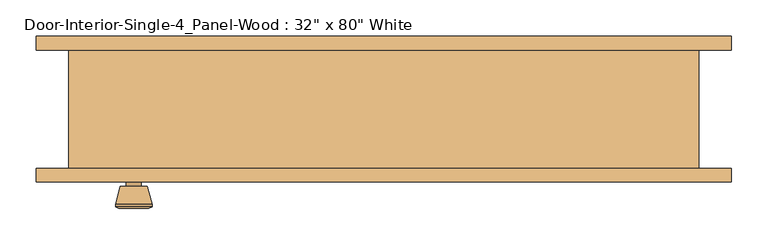
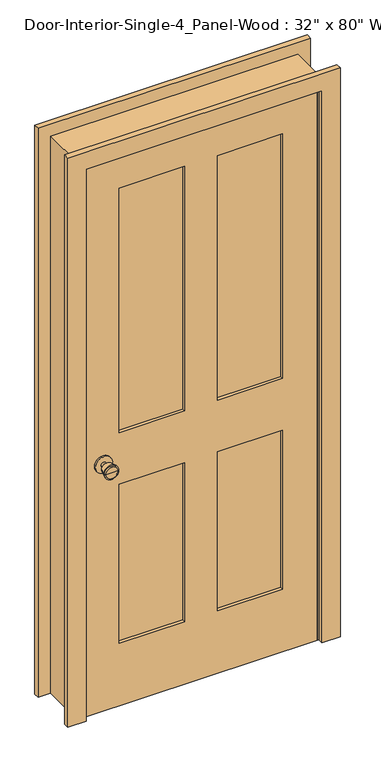
"""IFC4 building model written with IfcOpenShell, lengths in millimetres: door geometry."""

from ifc_helpers import new_model, si_unit, point, frame, frame_2d, origin, place, context, project, spatial, polyline, circle_curve, trimmed, segment, composite_curve, outline, extrude, faceted_brep, source, transform, mapped, element, save
from ifc_brep_helpers import plane_surface, cylinder_surface, revolved_surface, advanced_brep


def door_564574e5(model_context):
    return source(origin(), model_context, "Body", "SolidModel", [
        advanced_brep(
        [(-342.9, -36.8625, 914.4), (-352.9, -36.8625, 914.4), (-332.9, -36.8625, 914.4), (-322.4241324, 12.1375, 914.4), (-363.3758676, 12.1375, 914.4), (-342.9, 12.1375, 914.4), (-317.9, 10.3096319, 914.4), (-367.9, 10.3096319, 914.4), (-317.9, 6.8459537, 914.4), (-367.9, 6.8459537, 914.4), (-324.263764, -17.8625, 914.4), (-361.536236, -17.8625, 914.4), (-332.9, -17.8625, 914.4), (-352.9, -17.8625, 914.4)],
        [
            (0, 1),
            (1, 2, circle_curve(frame((-342.9, -36.8625, 914.4), z_axis=(0.0, -1.0, 0.0), x_axis=(-1.0, 0.0, 0.0)), 10.0)),
            (2, 0),
            (2, 1, circle_curve(frame((-342.9, -36.8625, 914.4), z_axis=(0.0, -1.0, 0.0), x_axis=(-1.0, 0.0, 0.0)), 10.0)),
            (3, 4, circle_curve(frame((-342.9, 12.1375, 914.4), z_axis=(0.0, 1.0, 0.0), x_axis=(-1.0, 0.0, 0.0)), 20.4758676)),
            (4, 5),
            (5, 3),
            (4, 3, circle_curve(frame((-342.9, 12.1375, 914.4), z_axis=(0.0, 1.0, 0.0), x_axis=(-1.0, 0.0, 0.0)), 20.4758676)),
            (6, 7, circle_curve(frame((-342.9, 10.3096319, 914.4), z_axis=(0.0, 1.0, 0.0), x_axis=(-1.0, 0.0, 0.0)), 25.0)),
            (7, 4),
            (3, 6),
            (7, 6, circle_curve(frame((-342.9, 10.3096319, 914.4), z_axis=(0.0, 1.0, 0.0), x_axis=(-1.0, 0.0, 0.0)), 25.0)),
            (8, 9, circle_curve(frame((-342.9, 6.8459537, 914.4), z_axis=(0.0, 1.0, 0.0), x_axis=(-1.0, 0.0, 0.0)), 25.0)),
            (9, 7),
            (6, 8),
            (9, 8, circle_curve(frame((-342.9, 6.8459537, 914.4), z_axis=(0.0, 1.0, 0.0), x_axis=(-1.0, 0.0, 0.0)), 25.0)),
            (10, 11, circle_curve(frame((-342.9, -17.8625, 914.4), z_axis=(0.0, 1.0, 0.0), x_axis=(-1.0, 0.0, 0.0)), 18.636236)),
            (11, 9),
            (8, 10),
            (11, 10, circle_curve(frame((-342.9, -17.8625, 914.4), z_axis=(0.0, 1.0, 0.0), x_axis=(-1.0, 0.0, 0.0)), 18.636236)),
            (12, 13, circle_curve(frame((-342.9, -17.8625, 914.4), z_axis=(0.0, 1.0, 0.0), x_axis=(-1.0, 0.0, 0.0)), 10.0)),
            (13, 11),
            (10, 12),
            (13, 12, circle_curve(frame((-342.9, -17.8625, 914.4), z_axis=(0.0, 1.0, 0.0), x_axis=(-1.0, 0.0, 0.0)), 10.0)),
            (1, 13),
            (12, 2),
        ],
        [
            plane_surface(frame((-342.9, -36.8625, 914.4), z_axis=(0.0, -1.0, 0.0), x_axis=(-1.0, 0.0, 0.0))),
            plane_surface(frame((-342.9, 12.1375, 914.4), z_axis=(0.0, 1.0, 0.0), x_axis=(-1.0, 0.0, 0.0))),
            revolved_surface(polyline([(-363.3758676, 12.1375, 914.4), (-367.9, 10.3096319, 914.4)]), (-342.9, -36.8625, 914.4), (0.0, -1.0, 0.0)),
            cylinder_surface(frame((-342.9, -36.8625, 914.4), z_axis=(0.0, -1.0, 0.0), x_axis=(-1.0, 0.0, 0.0)), 25.0),
            revolved_surface(polyline([(-367.9, 6.8459537, 914.4), (-361.536236, -17.8625, 914.4)]), (-342.9, -36.8625, 914.4), (0.0, -1.0, 0.0)),
            plane_surface(frame((-342.9, -17.8625, 914.4), z_axis=(0.0, -1.0, 0.0), x_axis=(-1.0, 0.0, 0.0))),
            cylinder_surface(frame((-342.9, -36.8625, 914.4), z_axis=(0.0, -1.0, 0.0), x_axis=(-1.0, 0.0, 0.0)), 10.0),
        ],
        [
            (0, [[1, 2, 3]]),
            (0, [[-3, 4, -1]]),
            (1, [[5, 6, 7]]),
            (1, [[8, -7, -6]]),
            (2, [[9, 10, -5, 11]]),
            (2, [[12, -11, -8, -10]]),
            (3, [[13, 14, -9, 15]]),
            (3, [[16, -15, -12, -14]]),
            (4, [[17, 18, -13, 19]]),
            (4, [[20, -19, -16, -18]]),
            (5, [[21, 22, -17, 23]]),
            (5, [[24, -23, -20, -22]]),
            (6, [[-2, 25, -21, 26]]),
            (6, [[-4, -26, -24, -25]]),
        ],
    ),
        extrude(outline(composite_curve([segment(trimmed(circle_curve(frame_2d((914.4, -342.9)), 30.0), [point((914.4, -372.9))], [point((914.4, -312.9))], False, "CARTESIAN"), True, "CONTINUOUS"), segment(trimmed(circle_curve(frame_2d((914.4, -342.9)), 30.0), [point((914.4, -312.9))], [point((914.4, -372.9))], False, "CARTESIAN"), True, "CONTINUOUS")], self_intersect=False)), frame((0.0, -42.8625, 0.0), z_axis=(0.0, 1.0, 0.0), x_axis=(0.0, 0.0, 1.0)), (0.0, 0.0, 1.0), 6.0),
        advanced_brep(
        [(-342.9, -83.7875, 914.4), (-332.9, -83.7875, 914.4), (-352.9, -83.7875, 914.4), (-322.4241324, -132.7875, 914.4), (-342.9, -132.7875, 914.4), (-363.3758676, -132.7875, 914.4), (-317.9, -130.9596319, 914.4), (-367.9, -130.9596319, 914.4), (-317.9, -127.4959537, 914.4), (-367.9, -127.4959537, 914.4), (-324.263764, -102.7875, 914.4), (-361.536236, -102.7875, 914.4), (-332.9, -102.7875, 914.4), (-352.9, -102.7875, 914.4)],
        [
            (0, 1),
            (1, 2, circle_curve(frame((-342.9, -83.7875, 914.4), z_axis=(0.0, 1.0, 0.0), x_axis=(-1.0, 0.0, 0.0)), 10.0)),
            (2, 0),
            (2, 1, circle_curve(frame((-342.9, -83.7875, 914.4), z_axis=(0.0, 1.0, 0.0), x_axis=(-1.0, 0.0, 0.0)), 10.0)),
            (3, 4),
            (4, 5),
            (5, 3, circle_curve(frame((-342.9, -132.7875, 914.4), z_axis=(0.0, -1.0, 0.0), x_axis=(-1.0, 0.0, 0.0)), 20.4758676)),
            (3, 5, circle_curve(frame((-342.9, -132.7875, 914.4), z_axis=(0.0, -1.0, 0.0), x_axis=(-1.0, 0.0, 0.0)), 20.4758676)),
            (6, 3),
            (5, 7),
            (7, 6, circle_curve(frame((-342.9, -130.9596319, 914.4), z_axis=(0.0, -1.0, 0.0), x_axis=(-1.0, 0.0, 0.0)), 25.0)),
            (6, 7, circle_curve(frame((-342.9, -130.9596319, 914.4), z_axis=(0.0, -1.0, 0.0), x_axis=(-1.0, 0.0, 0.0)), 25.0)),
            (8, 6),
            (7, 9),
            (9, 8, circle_curve(frame((-342.9, -127.4959537, 914.4), z_axis=(0.0, -1.0, 0.0), x_axis=(-1.0, 0.0, 0.0)), 25.0)),
            (8, 9, circle_curve(frame((-342.9, -127.4959537, 914.4), z_axis=(0.0, -1.0, 0.0), x_axis=(-1.0, 0.0, 0.0)), 25.0)),
            (10, 8),
            (9, 11),
            (11, 10, circle_curve(frame((-342.9, -102.7875, 914.4), z_axis=(0.0, -1.0, 0.0), x_axis=(-1.0, 0.0, 0.0)), 18.636236)),
            (10, 11, circle_curve(frame((-342.9, -102.7875, 914.4), z_axis=(0.0, -1.0, 0.0), x_axis=(-1.0, 0.0, 0.0)), 18.636236)),
            (12, 10),
            (11, 13),
            (13, 12, circle_curve(frame((-342.9, -102.7875, 914.4), z_axis=(0.0, -1.0, 0.0), x_axis=(-1.0, 0.0, 0.0)), 10.0)),
            (12, 13, circle_curve(frame((-342.9, -102.7875, 914.4), z_axis=(0.0, -1.0, 0.0), x_axis=(-1.0, 0.0, 0.0)), 10.0)),
            (1, 12),
            (13, 2),
        ],
        [
            plane_surface(frame((-342.9, -83.7875, 914.4), z_axis=(0.0, 1.0, 0.0), x_axis=(-1.0, 0.0, 0.0))),
            plane_surface(frame((-342.9, -132.7875, 914.4), z_axis=(0.0, -1.0, 0.0), x_axis=(-1.0, 0.0, 0.0))),
            revolved_surface(polyline([(-363.3758676, -132.7875, 914.4), (-367.9, -130.9596319, 914.4)]), (-342.9, -83.7875, 914.4), (0.0, 1.0, 0.0)),
            cylinder_surface(frame((-342.9, -83.7875, 914.4), z_axis=(0.0, 1.0, 0.0), x_axis=(-1.0, 0.0, 0.0)), 25.0),
            revolved_surface(polyline([(-367.9, -127.4959537, 914.4), (-361.536236, -102.7875, 914.4)]), (-342.9, -83.7875, 914.4), (0.0, 1.0, 0.0)),
            plane_surface(frame((-342.9, -102.7875, 914.4), z_axis=(0.0, 1.0, 0.0), x_axis=(-1.0, 0.0, 0.0))),
            cylinder_surface(frame((-342.9, -83.7875, 914.4), z_axis=(0.0, 1.0, 0.0), x_axis=(-1.0, 0.0, 0.0)), 10.0),
        ],
        [
            (0, [[1, 2, 3]]),
            (0, [[-3, 4, -1]]),
            (1, [[5, 6, 7]]),
            (1, [[-6, -5, 8]]),
            (2, [[9, -7, 10, 11]]),
            (2, [[-10, -8, -9, 12]]),
            (3, [[13, -11, 14, 15]]),
            (3, [[-14, -12, -13, 16]]),
            (4, [[17, -15, 18, 19]]),
            (4, [[-18, -16, -17, 20]]),
            (5, [[21, -19, 22, 23]]),
            (5, [[-22, -20, -21, 24]]),
            (6, [[25, -23, 26, -2]]),
            (6, [[-26, -24, -25, -4]]),
        ],
    ),
        extrude(outline(composite_curve([segment(trimmed(circle_curve(frame_2d((914.4, -342.9)), 30.0), [point((914.4, -372.9))], [point((914.4, -312.9))], False, "CARTESIAN"), True, "CONTINUOUS"), segment(trimmed(circle_curve(frame_2d((914.4, -342.9)), 30.0), [point((914.4, -312.9))], [point((914.4, -372.9))], False, "CARTESIAN"), True, "CONTINUOUS")], self_intersect=False)), frame((0.0, -83.7875, 0.0), z_axis=(0.0, 1.0, 0.0), x_axis=(0.0, 0.0, 1.0)), (0.0, 0.0, 1.0), 6.0),
        extrude(outline(polyline([(285.75, -54.5041667), (285.75, -66.1458333), (57.15, -66.1458333), (57.15, -54.5041667), (285.75, -54.5041667)])), frame((0.0, 0.0, 1009.65), z_axis=(0.0, 0.0, 1.0), x_axis=(1.0, 0.0, 0.0)), (0.0, 0.0, 1.0), 903.2875),
        extrude(outline(polyline([(-57.15, -54.5041667), (-57.15, -66.1458333), (-285.75, -66.1458333), (-285.75, -54.5041667), (-57.15, -54.5041667)])), frame((0.0, 0.0, 1009.65), z_axis=(0.0, 0.0, 1.0), x_axis=(1.0, 0.0, 0.0)), (0.0, 0.0, 1.0), 903.2875),
        extrude(outline(polyline([(285.75, -54.5041667), (285.75, -66.1458333), (57.15, -66.1458333), (57.15, -54.5041667), (285.75, -54.5041667)])), frame((0.0, 0.0, 231.775), z_axis=(0.0, 0.0, 1.0), x_axis=(1.0, 0.0, 0.0)), (0.0, 0.0, 1.0), 587.375),
        extrude(outline(polyline([(-57.15, -54.5041667), (-57.15, -66.1458333), (-285.75, -66.1458333), (-285.75, -54.5041667), (-57.15, -54.5041667)])), frame((0.0, 0.0, 231.775), z_axis=(0.0, 0.0, 1.0), x_axis=(1.0, 0.0, 0.0)), (0.0, 0.0, 1.0), 587.375),
        extrude(outline(polyline([(2032.0, -406.4), (0.0, -406.4), (0.0, 406.4), (2032.0, 406.4), (2032.0, -406.4)]), holes=[polyline([(1912.9375, 57.15), (1912.9375, 285.75), (1009.65, 285.75), (1009.65, 57.15), (1912.9375, 57.15)]), polyline([(1009.65, -57.15), (1009.65, -285.75), (1912.9375, -285.75), (1912.9375, -57.15), (1009.65, -57.15)]), polyline([(819.15, 57.15), (819.15, 285.75), (231.775, 285.75), (231.775, 57.15), (819.15, 57.15)]), polyline([(231.775, -57.15), (231.775, -285.75), (819.15, -285.75), (819.15, -57.15), (231.775, -57.15)])]), frame((0.0, -77.7875, 0.0), z_axis=(0.0, 1.0, 0.0), x_axis=(0.0, 0.0, 1.0)), (0.0, 0.0, 1.0), 34.925),
        faceted_brep([(431.8, -77.7875, 0.0), (406.4, -77.7875, 0.0), (406.4, -42.8625, 0.0), (393.7, -42.8625, 0.0), (393.7, -7.9375, 0.0), (406.4, -7.9375, 0.0), (406.4, 84.1375, 0.0), (431.8, 84.1375, 0.0), (431.8, 84.1375, 2057.4), (431.8, -77.7875, 2057.4), (406.4, 84.1375, 2032.0), (-406.4, 84.1375, 2032.0), (-406.4, 84.1375, 0.0), (-431.8, 84.1375, 0.0), (-431.8, 84.1375, 2057.4), (406.4, -7.9375, 2032.0), (393.7, -7.9375, 2019.3), (-393.7, -7.9375, 2019.3), (-393.7, -7.9375, 0.0), (-406.4, -7.9375, 0.0), (-406.4, -7.9375, 2032.0), (393.7, -42.8625, 2019.3), (406.4, -42.8625, 2032.0), (-406.4, -42.8625, 2032.0), (-406.4, -42.8625, 0.0), (-393.7, -42.8625, 0.0), (-393.7, -42.8625, 2019.3), (406.4, -77.7875, 2032.0), (-431.8, -77.7875, 2057.4), (-431.8, -77.7875, 0.0), (-406.4, -77.7875, 0.0), (-406.4, -77.7875, 2032.0)], [[[0, 1, 2, 3, 4, 5, 6, 7]], [[7, 8, 9, 0]], [[6, 10, 11, 12, 13, 14, 8, 7]], [[5, 15, 10, 6]], [[4, 16, 17, 18, 19, 20, 15, 5]], [[3, 21, 16, 4]], [[2, 22, 23, 24, 25, 26, 21, 3]], [[1, 27, 22, 2]], [[0, 9, 28, 29, 30, 31, 27, 1]], [[8, 14, 28, 9]], [[15, 20, 11, 10]], [[21, 26, 17, 16]], [[27, 31, 23, 22]], [[29, 13, 12, 19, 18, 25, 24, 30]], [[14, 13, 29, 28]], [[20, 19, 12, 11]], [[26, 25, 18, 17]], [[31, 30, 24, 23]]]),
        extrude(outline(polyline([(0.0, 476.25), (2101.85, 476.25), (2101.85, -476.25), (0.0, -476.25), (0.0, -412.75), (2038.35, -412.75), (2038.35, 412.75), (0.0, 412.75), (0.0, 476.25)])), frame((0.0, 84.1375, 0.0), z_axis=(0.0, 1.0, 0.0), x_axis=(0.0, 0.0, 1.0)), (0.0, 0.0, 1.0), 19.05),
        extrude(outline(polyline([(0.0, 476.25), (2101.85, 476.25), (2101.85, -476.25), (0.0, -476.25), (0.0, -412.75), (2038.35, -412.75), (2038.35, 412.75), (0.0, 412.75), (0.0, 476.25)])), frame((0.0, -96.8375, 0.0), z_axis=(0.0, 1.0, 0.0), x_axis=(0.0, 0.0, 1.0)), (0.0, 0.0, 1.0), 19.05),
    ])


if __name__ == "__main__":
    model = new_model("IFC4")
    model_context = context("Model", 3, world=origin())
    ifc_project = project(units=[si_unit("LENGTHUNIT", "METRE", prefix="MILLI")], contexts=[model_context])
    site = spatial("IfcSite", under=ifc_project)
    building = spatial("IfcBuilding", under=site)
    placement = place(None, origin())
    door_shape = door_564574e5(model_context)
    element("IfcDoor", 1, ObjectType="Door-Interior-Single-4_Panel-Wood : 32\" x 80\" White", at=placement, inside=building, context=model_context, shape_type="MappedRepresentation", body=[
        mapped(door_shape, transform((0.0, 0.0, 0.0), x_axis=(1.0, 0.0, 0.0), y_axis=(0.0, 1.0, 0.0), z_axis=(0.0, 0.0, 1.0))),
    ])
    save(model, "model.ifc")

# Revit data of these elements
# Type "Door-Interior-Single-4_Panel-Wood : 32\" x 80\" White"
#   Type Mark = "48"
#   COBie.Type.CreatedBy = "doug.wood@us.ibm.com"
#   COBie.Type.CreatedOn = "2016-04-14T02:07:24"
#   COBie.Type.Name = "Doors_Door-Interior-Single-4_Panel-Wood_32\" x 80\" White_48"
#   COBie.Type.Category = "23-30 10 00 : Doors"
#   COBie.Type.Description = "Door-Interior-Single-4_Panel-Wood_32\" x 80\" White"
#   COBie.Type.Manufacturer = ""
#   COBie.Type.ModelNumber = ""
#   Assembly Code = "C1020300"
#   Analytic Construction = "Wooden"
#   COBie.Type.ReplacementCost = 0
#   Top Rail = 0' - 4 11/16"
#   Thickness = 0' - 1 3/8"
#   Thermal Resistance (R) = 0.455703 (m²·K)/W
#   Swing Angle [instance default] = 90.00°
#   Stiles = 0' - 4 3/4"
#   Rough Width = 2' - 10"
#   Rough Height = 6' - 9"
#   Mullion = 0' - 4 1/2"
#   Lock Rail = 0' - 7 1/2"
#   Height = 6' - 8"
#   Width = 2' - 8"
#   Heat Transfer Coefficient (U) = 2.19465 W/(m²·K)
#   Bottom Rail = 0' - 9 1/8"
#   COBie.Type = no
#   Trim Material = Trim - White
#   Panel Material = Door - Panel - White
#   Frame Material = Door - Panel - White
#   Door Handle Material = ARCAT - Metal - Brass, Polished
#   Visual Light Transmittance = 0
#   Solar Heat Gain Coefficient = 0
#   Wall Closure = (empty or 0)
#   Function = (empty or 0)
# Element 1 (IfcDoor, "Door-Interior-Single-4_Panel-Wood : 32\" x 80\" White")
#   Materials on its faces: "Door - Panel - White", "ARCAT - Metal - Brass, Polished", "Trim - White"
# Materials
#   "Trim - White": class "Wood", colour RGB 255 255 255, transparency 0, Cost = 0
#   "Door - Panel - White": class "Wood", colour RGB 255 255 255, transparency 0, Cost = 0
#   "ARCAT - Metal - Brass, Polished": class "Unassigned", colour RGB 246 240 166, transparency 0, Keynote = "05050", Model = "Generic", Manufacturer = "Generic", Description = "Steel, Chrome Plated"
